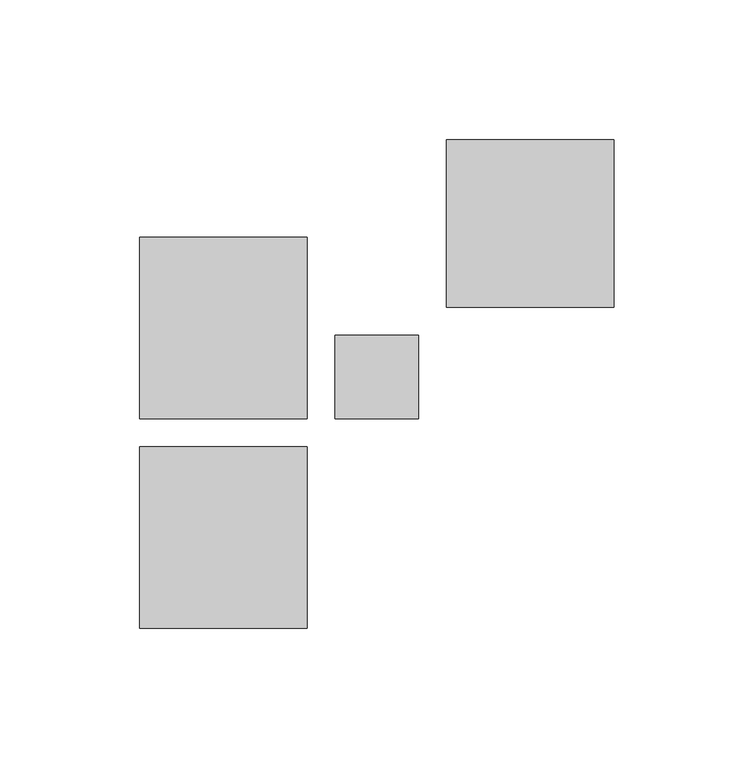
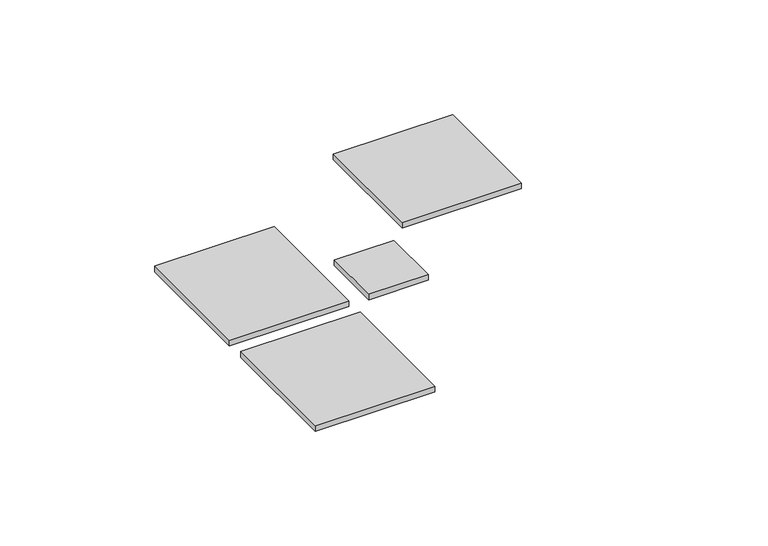
"""IFC4 building model written with IfcOpenShell, lengths in millimetres: proxy geometry, TSP Submersible Light Point : TSP Submersible Light Point."""

import ifcopenshell
import ifcopenshell.guid

model = None  # the IFC model being written
_history = None  # IfcOwnerHistory: only IFC2X3 demands one
_inside = {}  # id of a spatial element -> (the spatial element, [elements in it])
_under = {}  # id of a project, library or spatial element -> (it, [spatial elements below it])
_declared = {}  # id of a project -> (the project, [libraries it declares])
_typed = {}  # id of a type object -> (the type object, [elements of that type])
_made_of = {}  # id of a material, layer set ... -> (it, [elements and type objects made of it])


def new_model(schema):
    """Start an empty IFC model of exactly this schema.

    Asked for "IFC4X3", IfcOpenShell would pick the latest addendum, in which some entities
    have other attributes; the version numbers below select the first issue.
    IFC2X3 requires an IfcOwnerHistory on every rooted entity: one is made here for all.
    """
    global model, _history
    if schema == "IFC4X3":
        model = ifcopenshell.file(schema_version=(4, 3, 0, 0))
    else:
        model = ifcopenshell.file(schema=schema)
    _inside.clear()
    _under.clear()
    _declared.clear()
    _typed.clear()
    _made_of.clear()
    _history = None
    if model.schema == "IFC2X3":
        org = make("IfcOrganization", Name="unknown")
        user = make(
            "IfcPersonAndOrganization",
            ThePerson=make("IfcPerson", FamilyName="unknown"),
            TheOrganization=org,
        )
        app = make(
            "IfcApplication",
            ApplicationDeveloper=org,
            Version="unknown",
            ApplicationFullName="unknown",
            ApplicationIdentifier="unknown",
        )
        _history = make(
            "IfcOwnerHistory",
            OwningUser=user,
            OwningApplication=app,
            ChangeAction="ADDED",
            CreationDate=0,
        )
    return model


def make(cls, **values):
    """One entity of the class cls with the attributes given. An attribute that is None is left unset."""
    return model.create_entity(
        cls, **{name: value for name, value in values.items() if value is not None}
    )


def rooted(cls, **values):
    """An entity with a GlobalId (a new one), such as an element, a storey or a relation."""
    return make(cls, GlobalId=ifcopenshell.guid.new(), OwnerHistory=_history, **values)


def si_unit(unit_type, name, prefix=None):
    """IfcSIUnit, for example si_unit("LENGTHUNIT", "METRE", prefix="MILLI")."""
    return make("IfcSIUnit", UnitType=unit_type, Prefix=prefix, Name=name)


def assignment(units):
    """IfcUnitAssignment: the units of a project."""
    return None if units is None else make("IfcUnitAssignment", Units=units)


def point(xyz):
    """IfcCartesianPoint."""
    return None if xyz is None else make("IfcCartesianPoint", Coordinates=xyz)


def direction(xyz):
    """IfcDirection."""
    return None if xyz is None else make("IfcDirection", DirectionRatios=xyz)


def frame(location, z_axis=None, x_axis=None):
    """IfcAxis2Placement3D, a coordinate frame: its origin and axes. An axis left out is left unset."""
    return make(
        "IfcAxis2Placement3D",
        Location=point(location),
        Axis=direction(z_axis),
        RefDirection=direction(x_axis),
    )


def origin():
    """The frame at (0, 0, 0) with its axes left unset."""
    return frame((0.0, 0.0, 0.0))


def origin_with_axes():
    """The frame at (0, 0, 0) with the z axis (0, 0, 1) and the x axis (1, 0, 0) written out."""
    return frame((0.0, 0.0, 0.0), z_axis=(0.0, 0.0, 1.0), x_axis=(1.0, 0.0, 0.0))


def place(relative_to, where):
    """IfcLocalPlacement: puts the frame where relative to a parent placement (None: the world)."""
    return make(
        "IfcLocalPlacement", PlacementRelTo=relative_to, RelativePlacement=where
    )


def context(
    kind, dimensions, precision=None, world=None, true_north=None, identifier=None
):
    """IfcGeometricRepresentationContext, for example the 3D "Model" context."""
    return make(
        "IfcGeometricRepresentationContext",
        ContextIdentifier=identifier,
        ContextType=kind,
        CoordinateSpaceDimension=dimensions,
        Precision=precision,
        WorldCoordinateSystem=world,
        TrueNorth=true_north,
    )


def project(units=None, contexts=None):
    """IfcProject with its units and contexts."""
    return rooted(
        "IfcProject",
        Name="project",
        RepresentationContexts=contexts,
        UnitsInContext=assignment(units),
    )


def spatial(cls, under=None, at=None, **own):
    """A site, building, storey or space (cls), placed at a placement, below another one or the project."""
    s = rooted(cls, ObjectPlacement=at, **own)
    if under is not None:
        _under.setdefault(under.id(), (under, []))[1].append(s)
    return s


def polyline(points):
    """IfcPolyline through the points."""
    return make("IfcPolyline", Points=[point(p) for p in points])


def outline(outer, holes=None, kind="AREA"):
    """IfcArbitraryClosedProfileDef: a profile drawn as a closed curve; with holes, ...WithVoids."""
    if holes is None:
        return make("IfcArbitraryClosedProfileDef", ProfileType=kind, OuterCurve=outer)
    return make(
        "IfcArbitraryProfileDefWithVoids",
        ProfileType=kind,
        OuterCurve=outer,
        InnerCurves=holes,
    )


def extrude(swept, where, along, depth):
    """IfcExtrudedAreaSolid: the profile swept, set in the frame where, extruded along a direction by depth."""
    return make(
        "IfcExtrudedAreaSolid",
        SweptArea=swept,
        Position=where,
        ExtrudedDirection=direction(along),
        Depth=depth,
    )


def shape(context_of_items, identifier, shape_type, items):
    """IfcShapeRepresentation: the items that make up one representation, for example the "Body"."""
    return make(
        "IfcShapeRepresentation",
        ContextOfItems=context_of_items,
        RepresentationIdentifier=identifier,
        RepresentationType=shape_type,
        Items=items,
    )


def source(mapping_origin, context_of_items, identifier, shape_type, items):
    """IfcRepresentationMap: a shape defined once, which mapped items show again and again."""
    return make(
        "IfcRepresentationMap",
        MappingOrigin=mapping_origin,
        MappedRepresentation=shape(context_of_items, identifier, shape_type, items),
    )


def transform(
    local_origin,
    x_axis=None,
    y_axis=None,
    z_axis=None,
    scale=None,
    scale2=None,
    scale3=None,
    uniform=True,
):
    """IfcCartesianTransformationOperator3D, or its non-uniform kind. x_axis, y_axis, z_axis: its Axis1, 2, 3."""
    if uniform:
        return make(
            "IfcCartesianTransformationOperator3D",
            Axis1=direction(x_axis),
            Axis2=direction(y_axis),
            LocalOrigin=point(local_origin),
            Scale=scale,
            Axis3=direction(z_axis),
        )
    return make(
        "IfcCartesianTransformationOperator3DnonUniform",
        Axis1=direction(x_axis),
        Axis2=direction(y_axis),
        LocalOrigin=point(local_origin),
        Scale=scale,
        Axis3=direction(z_axis),
        Scale2=scale2,
        Scale3=scale3,
    )


def mapped(mapping_source, mapping_target):
    """IfcMappedItem: shows the shape of a source again, moved by a transform."""
    return make(
        "IfcMappedItem", MappingSource=mapping_source, MappingTarget=mapping_target
    )


def made_of(thing, what):
    """Note that an element or type object is made of a material, layer set ...; save() writes the relation."""
    if what is not None:
        _made_of.setdefault(what.id(), (what, []))[1].append(thing)
    return thing


def element(
    cls,
    number,
    at=None,
    inside=None,
    cuts=None,
    type_object=None,
    material=None,
    context=None,
    identifier="Body",
    shape_type=None,
    held_by="IfcProductDefinitionShape",
    body=None,
    shapes=None,
    **own,
):
    """One element of the class cls, such as IfcWall. Its Tag is "e" and its number.

    at: its placement. inside: the storey or other place that contains it. cuts: it is an
    opening in that element (IfcRelVoidsElement). A single representation is given by context,
    identifier, shape_type and body (its items); several are given by shapes. held_by: the class
    of the entity that holds the representations. save() writes the other relations.
    """
    e = rooted(cls, Tag="e%d" % number, ObjectPlacement=at, **own)
    if body is not None:
        shapes = [shape(context, identifier, shape_type, body)]
    if shapes is not None:
        e.Representation = make(held_by, Representations=shapes)
    if inside is not None:
        _inside.setdefault(inside.id(), (inside, []))[1].append(e)
    if cuts is not None:
        rooted(
            "IfcRelVoidsElement", RelatingBuildingElement=cuts, RelatedOpeningElement=e
        )
    if type_object is not None:
        _typed.setdefault(type_object.id(), (type_object, []))[1].append(e)
    return made_of(e, material)


def aggregate(whole, parts):
    """IfcRelAggregates: a whole, such as a stair, and the parts it consists of."""
    return rooted("IfcRelAggregates", RelatingObject=whole, RelatedObjects=parts)


def save(model, path):
    """Write the relations noted so far, then the file.

    IfcRelAggregates (storeys below a building ...), IfcRelContainedInSpatialStructure (elements
    in a storey), IfcRelDefinesByType, IfcRelAssociatesMaterial and IfcRelDeclares: one each for
    every whole, place, type object, material and project.
    """
    for whole, parts in _under.values():
        aggregate(whole, parts)
    for where, things in _inside.values():
        rooted(
            "IfcRelContainedInSpatialStructure",
            RelatedElements=things,
            RelatingStructure=where,
        )
    for kind, things in _typed.values():
        rooted("IfcRelDefinesByType", RelatedObjects=things, RelatingType=kind)
    for what, things in _made_of.values():
        rooted("IfcRelAssociatesMaterial", RelatedObjects=things, RelatingMaterial=what)
    for by, libraries in _declared.values():
        rooted("IfcRelDeclares", RelatingContext=by, RelatedDefinitions=libraries)
    model.write(path)


def electrical_fixtures_57553e7b(model_context):
    return source(origin(), model_context, "Body", "SweptSolid", [
        extrude(outline(polyline([(-65.0, -5.0), (-5.0, -5.0), (-5.0, -70.0), (-65.0, -70.0), (-65.0, -5.0)])), origin_with_axes(), (0.0, 0.0, 1.0), 3.0),
        extrude(outline(polyline([(35.0, 5.0), (5.0, 5.0), (5.0, 35.0), (35.0, 35.0), (35.0, 5.0)])), origin_with_axes(), (0.0, 0.0, 1.0), 3.0),
        extrude(outline(polyline([(105.0, 45.0), (45.0, 45.0), (45.0, 105.0), (105.0, 105.0), (105.0, 45.0)])), origin_with_axes(), (0.0, 0.0, 1.0), 3.0),
        extrude(outline(polyline([(-65.0, 5.0), (-65.0, 70.0), (-5.0, 70.0), (-5.0, 5.0), (-65.0, 5.0)])), origin_with_axes(), (0.0, 0.0, 1.0), 3.0),
    ])


if __name__ == "__main__":
    model = new_model("IFC4")
    model_context = context("Model", 3, world=origin())
    ifc_project = project(units=[si_unit("LENGTHUNIT", "METRE", prefix="MILLI")], contexts=[model_context])
    site = spatial("IfcSite", under=ifc_project)
    building = spatial("IfcBuilding", under=site)
    placement = place(None, origin())
    electrical_fixtures_shape = electrical_fixtures_57553e7b(model_context)
    element("IfcBuildingElementProxy", 1, Name="TSP Submersible Light Point : TSP Submersible Light Point", ObjectType="TSP Submersible Light Point : TSP Submersible Light Point", at=placement, inside=building, context=model_context, shape_type="MappedRepresentation", body=[
        mapped(electrical_fixtures_shape, transform((0.0, 0.0, 0.0), x_axis=(1.0, 0.0, 0.0), y_axis=(0.0, 1.0, 0.0), z_axis=(0.0, 0.0, 1.0))),
    ])
    save(model, "model.ifc")

# Revit data of these elements
# Type "TSP Submersible Light Point : TSP Submersible Light Point"
#   Model = "TSP_ELEC220SUBLP"
#   Default Elevation = 0
# Element 1 (IfcBuildingElementProxy, "TSP Submersible Light Point : TSP Submersible Light Point")
#   Materials on its faces: "Plastic, Opaque Black"
# Materials
#   "Plastic, Opaque Black": class "Plastic", colour RGB 0 0 0, transparency 0.7, Description = "Plastic, generic, opaque black", Cost = 0
